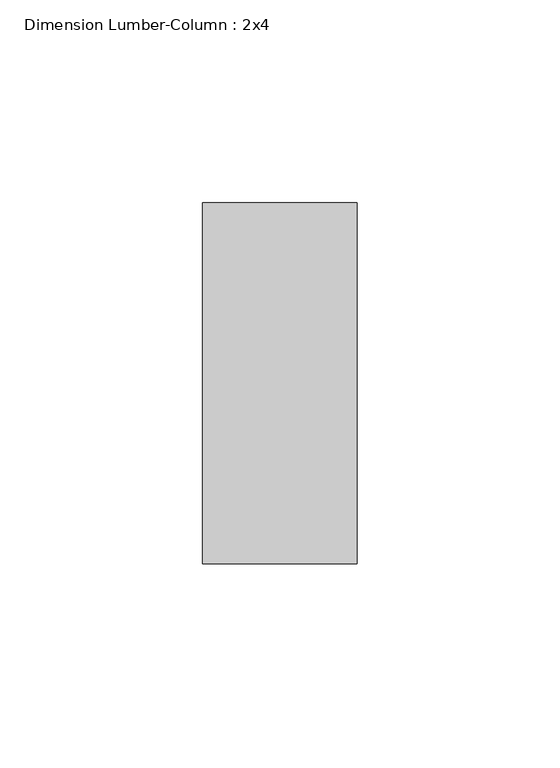
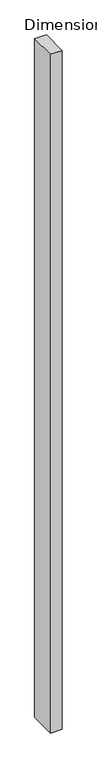
"""IFC4 building model written with IfcOpenShell, lengths in millimetres: column geometry, Dimension Lumber-Column : 2x4."""

from ifc_helpers import new_model, si_unit, frame, origin, place, context, project, spatial, polyline, outline, extrude, source, transform, mapped, element, save


def dimension_lumber_column_2x4_ae31bb9f(model_context):
    return source(origin(), model_context, "Body", "SweptSolid", [
        extrude(outline(polyline([(19.05, 44.45), (19.05, -44.45), (-19.05, -44.45), (-19.05, 44.45), (19.05, 44.45)])), frame((0.0, 0.0, 56.35625), z_axis=(0.0, 0.0, 1.0), x_axis=(1.0, 0.0, 0.0)), (0.0, 0.0, 1.0), 2331.24375),
    ])


if __name__ == "__main__":
    model = new_model("IFC4")
    model_context = context("Model", 3, world=origin())
    ifc_project = project(units=[si_unit("LENGTHUNIT", "METRE", prefix="MILLI")], contexts=[model_context])
    site = spatial("IfcSite", under=ifc_project)
    building = spatial("IfcBuilding", under=site)
    placement = place(None, origin())
    dimension_lumber_column_2x4_shape = dimension_lumber_column_2x4_ae31bb9f(model_context)
    element("IfcColumn", 1, ObjectType="Dimension Lumber-Column : 2x4", at=placement, inside=building, context=model_context, shape_type="MappedRepresentation", body=[
        mapped(dimension_lumber_column_2x4_shape, transform((0.0, 0.0, 0.0), x_axis=(1.0, 0.0, 0.0), y_axis=(0.0, 1.0, 0.0), z_axis=(0.0, 0.0, 1.0))),
    ])
    save(model, "model.ifc")

# Revit data of these elements
# Type "Dimension Lumber-Column : 2x4"
#   Int Type = "Interior"
#   Assembly Code = "B10"
#   Cost = 8.05
#   A = 0.0364583 SF
#   b = 0' - 1 1/2"
#   d = 0' - 3 1/2"
#   Structural Material [instance default] = Softwood, Lumber
# Element 1 (IfcColumn, "Dimension Lumber-Column : 2x4")
#   Structural Material = Douglas Fir #2
#   Materials on its faces: "Douglas Fir #2"
# Materials
#   "Softwood, Lumber": class "Wood", colour RGB 223 192 134, transparency 0, Description = "Pinus Echinata", Cost = 0
#   "Douglas Fir #2": class "Wood", colour RGB 223 192 134, transparency 0, Description = "Pinus Echinata", Cost = 0
